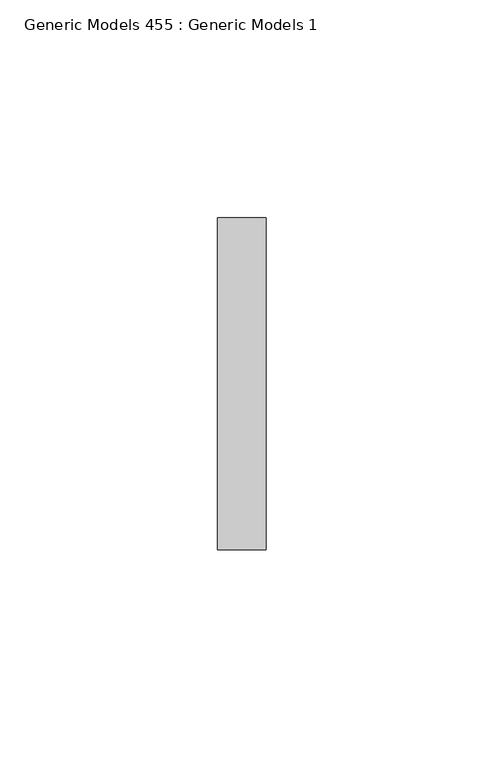
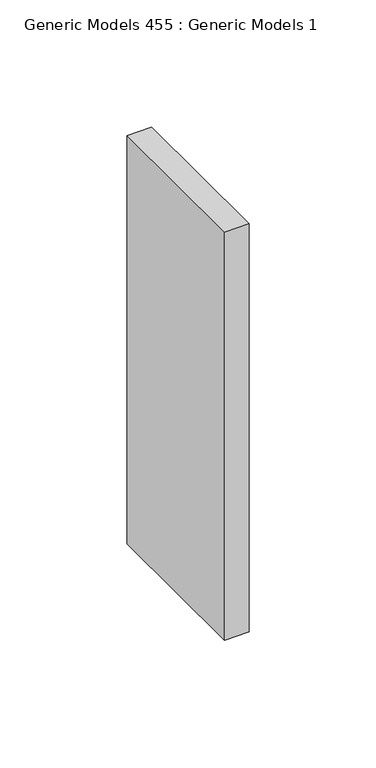
"""IFC4 building model written with IfcOpenShell, lengths in millimetres: proxy geometry, Generic Models 455 : Generic Models 1."""

from ifc_helpers import new_model, si_unit, frame, origin, place, context, project, spatial, polyline, outline, extrude, source, transform, mapped, element, save


def generic_models_455_generic_models_1_05fa7ba1(model_context):
    return source(origin(), model_context, "Body", "SweptSolid", [
        extrude(outline(polyline([(1642.0050572, 4604.9120715), (1653.1175572, 4604.9120715), (1653.1175572, 4528.7120715), (1642.0050572, 4528.7120715), (1642.0050572, 4604.9120715)])), frame((0.0, 0.0, 129219.3267146), z_axis=(0.0, 0.0, 1.0), x_axis=(1.0, 0.0, 0.0)), (0.0, 0.0, 1.0), 195.7003824),
    ])


if __name__ == "__main__":
    model = new_model("IFC4")
    model_context = context("Model", 3, world=origin())
    ifc_project = project(units=[si_unit("LENGTHUNIT", "METRE", prefix="MILLI")], contexts=[model_context])
    site = spatial("IfcSite", under=ifc_project)
    building = spatial("IfcBuilding", under=site)
    placement = place(None, origin())
    generic_models_455_generic_models_1_shape = generic_models_455_generic_models_1_05fa7ba1(model_context)
    element("IfcBuildingElementProxy", 1, Name="Generic Models 455 : Generic Models 1", ObjectType="Generic Models 455 : Generic Models 1", at=placement, inside=building, context=model_context, shape_type="MappedRepresentation", body=[
        mapped(generic_models_455_generic_models_1_shape, transform((0.0, 0.0, 0.0), x_axis=(1.0, 0.0, 0.0), y_axis=(0.0, 1.0, 0.0), z_axis=(0.0, 0.0, 1.0))),
    ])
    save(model, "model.ifc")

# Revit data of these elements
# Element 1 (IfcBuildingElementProxy, "Generic Models 455 : Generic Models 1")
#   Materials on its faces: "_VERTICAL BATTEN STRIPS - COR-A-VENT - 7/16\" X 3\" - 16\" O.C. - (BEYOND)"
# Materials
#   "_VERTICAL BATTEN STRIPS - COR-A-VENT - 7/16\" X 3\" - 16\" O.C. - (BEYOND)": class "Generic", colour RGB 190 220 196, transparency 0, Cost = 0
